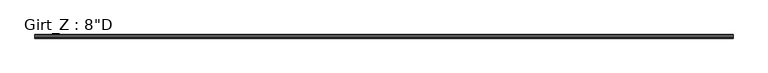
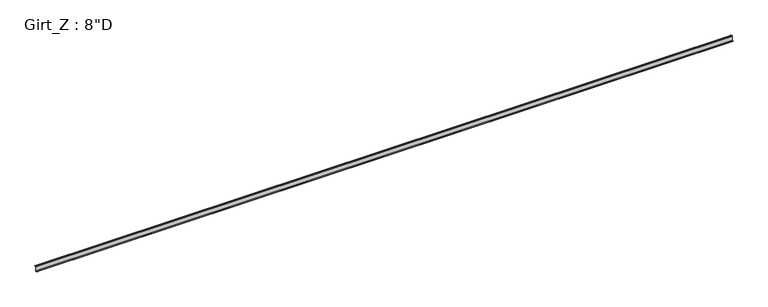
"""IFC4 building model written with IfcOpenShell, lengths in millimetres: beam geometry."""

import ifcopenshell
import ifcopenshell.guid

model = None  # the IFC model being written
_history = None  # IfcOwnerHistory: only IFC2X3 demands one
_inside = {}  # id of a spatial element -> (the spatial element, [elements in it])
_under = {}  # id of a project, library or spatial element -> (it, [spatial elements below it])
_declared = {}  # id of a project -> (the project, [libraries it declares])
_typed = {}  # id of a type object -> (the type object, [elements of that type])
_made_of = {}  # id of a material, layer set ... -> (it, [elements and type objects made of it])


def new_model(schema):
    """Start an empty IFC model of exactly this schema.

    Asked for "IFC4X3", IfcOpenShell would pick the latest addendum, in which some entities
    have other attributes; the version numbers below select the first issue.
    IFC2X3 requires an IfcOwnerHistory on every rooted entity: one is made here for all.
    """
    global model, _history
    if schema == "IFC4X3":
        model = ifcopenshell.file(schema_version=(4, 3, 0, 0))
    else:
        model = ifcopenshell.file(schema=schema)
    _inside.clear()
    _under.clear()
    _declared.clear()
    _typed.clear()
    _made_of.clear()
    _history = None
    if model.schema == "IFC2X3":
        org = make("IfcOrganization", Name="unknown")
        user = make(
            "IfcPersonAndOrganization",
            ThePerson=make("IfcPerson", FamilyName="unknown"),
            TheOrganization=org,
        )
        app = make(
            "IfcApplication",
            ApplicationDeveloper=org,
            Version="unknown",
            ApplicationFullName="unknown",
            ApplicationIdentifier="unknown",
        )
        _history = make(
            "IfcOwnerHistory",
            OwningUser=user,
            OwningApplication=app,
            ChangeAction="ADDED",
            CreationDate=0,
        )
    return model


def make(cls, **values):
    """One entity of the class cls with the attributes given. An attribute that is None is left unset."""
    return model.create_entity(
        cls, **{name: value for name, value in values.items() if value is not None}
    )


def rooted(cls, **values):
    """An entity with a GlobalId (a new one), such as an element, a storey or a relation."""
    return make(cls, GlobalId=ifcopenshell.guid.new(), OwnerHistory=_history, **values)


def si_unit(unit_type, name, prefix=None):
    """IfcSIUnit, for example si_unit("LENGTHUNIT", "METRE", prefix="MILLI")."""
    return make("IfcSIUnit", UnitType=unit_type, Prefix=prefix, Name=name)


def assignment(units):
    """IfcUnitAssignment: the units of a project."""
    return None if units is None else make("IfcUnitAssignment", Units=units)


def point(xyz):
    """IfcCartesianPoint."""
    return None if xyz is None else make("IfcCartesianPoint", Coordinates=xyz)


def direction(xyz):
    """IfcDirection."""
    return None if xyz is None else make("IfcDirection", DirectionRatios=xyz)


def frame(location, z_axis=None, x_axis=None):
    """IfcAxis2Placement3D, a coordinate frame: its origin and axes. An axis left out is left unset."""
    return make(
        "IfcAxis2Placement3D",
        Location=point(location),
        Axis=direction(z_axis),
        RefDirection=direction(x_axis),
    )


def frame_2d(location, x_axis=None):
    """IfcAxis2Placement2D, a coordinate frame in the plane: its origin and x axis."""
    return make(
        "IfcAxis2Placement2D", Location=point(location), RefDirection=direction(x_axis)
    )


def origin():
    """The frame at (0, 0, 0) with its axes left unset."""
    return frame((0.0, 0.0, 0.0))


def place(relative_to, where):
    """IfcLocalPlacement: puts the frame where relative to a parent placement (None: the world)."""
    return make(
        "IfcLocalPlacement", PlacementRelTo=relative_to, RelativePlacement=where
    )


def context(
    kind, dimensions, precision=None, world=None, true_north=None, identifier=None
):
    """IfcGeometricRepresentationContext, for example the 3D "Model" context."""
    return make(
        "IfcGeometricRepresentationContext",
        ContextIdentifier=identifier,
        ContextType=kind,
        CoordinateSpaceDimension=dimensions,
        Precision=precision,
        WorldCoordinateSystem=world,
        TrueNorth=true_north,
    )


def project(units=None, contexts=None):
    """IfcProject with its units and contexts."""
    return rooted(
        "IfcProject",
        Name="project",
        RepresentationContexts=contexts,
        UnitsInContext=assignment(units),
    )


def spatial(cls, under=None, at=None, **own):
    """A site, building, storey or space (cls), placed at a placement, below another one or the project."""
    s = rooted(cls, ObjectPlacement=at, **own)
    if under is not None:
        _under.setdefault(under.id(), (under, []))[1].append(s)
    return s


def polyline(points):
    """IfcPolyline through the points."""
    return make("IfcPolyline", Points=[point(p) for p in points])


def circle_curve(where, radius):
    """IfcCircle in the frame where."""
    return make("IfcCircle", Position=where, Radius=radius)


def trimmed(basis, trim1, trim2, sense, master):
    """IfcTrimmedCurve: the piece of a basis curve between two trims."""
    return make(
        "IfcTrimmedCurve",
        BasisCurve=basis,
        Trim1=trim1,
        Trim2=trim2,
        SenseAgreement=sense,
        MasterRepresentation=master,
    )


def segment(curve, same_sense, transition):
    """IfcCompositeCurveSegment."""
    return make(
        "IfcCompositeCurveSegment",
        Transition=transition,
        SameSense=same_sense,
        ParentCurve=curve,
    )


def composite_curve(segments, self_intersect=None):
    """IfcCompositeCurve: segments joined end to end."""
    return make("IfcCompositeCurve", Segments=segments, SelfIntersect=self_intersect)


def outline(outer, holes=None, kind="AREA"):
    """IfcArbitraryClosedProfileDef: a profile drawn as a closed curve; with holes, ...WithVoids."""
    if holes is None:
        return make("IfcArbitraryClosedProfileDef", ProfileType=kind, OuterCurve=outer)
    return make(
        "IfcArbitraryProfileDefWithVoids",
        ProfileType=kind,
        OuterCurve=outer,
        InnerCurves=holes,
    )


def extrude(swept, where, along, depth):
    """IfcExtrudedAreaSolid: the profile swept, set in the frame where, extruded along a direction by depth."""
    return make(
        "IfcExtrudedAreaSolid",
        SweptArea=swept,
        Position=where,
        ExtrudedDirection=direction(along),
        Depth=depth,
    )


def shape(context_of_items, identifier, shape_type, items):
    """IfcShapeRepresentation: the items that make up one representation, for example the "Body"."""
    return make(
        "IfcShapeRepresentation",
        ContextOfItems=context_of_items,
        RepresentationIdentifier=identifier,
        RepresentationType=shape_type,
        Items=items,
    )


def source(mapping_origin, context_of_items, identifier, shape_type, items):
    """IfcRepresentationMap: a shape defined once, which mapped items show again and again."""
    return make(
        "IfcRepresentationMap",
        MappingOrigin=mapping_origin,
        MappedRepresentation=shape(context_of_items, identifier, shape_type, items),
    )


def transform(
    local_origin,
    x_axis=None,
    y_axis=None,
    z_axis=None,
    scale=None,
    scale2=None,
    scale3=None,
    uniform=True,
):
    """IfcCartesianTransformationOperator3D, or its non-uniform kind. x_axis, y_axis, z_axis: its Axis1, 2, 3."""
    if uniform:
        return make(
            "IfcCartesianTransformationOperator3D",
            Axis1=direction(x_axis),
            Axis2=direction(y_axis),
            LocalOrigin=point(local_origin),
            Scale=scale,
            Axis3=direction(z_axis),
        )
    return make(
        "IfcCartesianTransformationOperator3DnonUniform",
        Axis1=direction(x_axis),
        Axis2=direction(y_axis),
        LocalOrigin=point(local_origin),
        Scale=scale,
        Axis3=direction(z_axis),
        Scale2=scale2,
        Scale3=scale3,
    )


def mapped(mapping_source, mapping_target):
    """IfcMappedItem: shows the shape of a source again, moved by a transform."""
    return make(
        "IfcMappedItem", MappingSource=mapping_source, MappingTarget=mapping_target
    )


def made_of(thing, what):
    """Note that an element or type object is made of a material, layer set ...; save() writes the relation."""
    if what is not None:
        _made_of.setdefault(what.id(), (what, []))[1].append(thing)
    return thing


def element(
    cls,
    number,
    at=None,
    inside=None,
    cuts=None,
    type_object=None,
    material=None,
    context=None,
    identifier="Body",
    shape_type=None,
    held_by="IfcProductDefinitionShape",
    body=None,
    shapes=None,
    **own,
):
    """One element of the class cls, such as IfcWall. Its Tag is "e" and its number.

    at: its placement. inside: the storey or other place that contains it. cuts: it is an
    opening in that element (IfcRelVoidsElement). A single representation is given by context,
    identifier, shape_type and body (its items); several are given by shapes. held_by: the class
    of the entity that holds the representations. save() writes the other relations.
    """
    e = rooted(cls, Tag="e%d" % number, ObjectPlacement=at, **own)
    if body is not None:
        shapes = [shape(context, identifier, shape_type, body)]
    if shapes is not None:
        e.Representation = make(held_by, Representations=shapes)
    if inside is not None:
        _inside.setdefault(inside.id(), (inside, []))[1].append(e)
    if cuts is not None:
        rooted(
            "IfcRelVoidsElement", RelatingBuildingElement=cuts, RelatedOpeningElement=e
        )
    if type_object is not None:
        _typed.setdefault(type_object.id(), (type_object, []))[1].append(e)
    return made_of(e, material)


def aggregate(whole, parts):
    """IfcRelAggregates: a whole, such as a stair, and the parts it consists of."""
    return rooted("IfcRelAggregates", RelatingObject=whole, RelatedObjects=parts)


def save(model, path):
    """Write the relations noted so far, then the file.

    IfcRelAggregates (storeys below a building ...), IfcRelContainedInSpatialStructure (elements
    in a storey), IfcRelDefinesByType, IfcRelAssociatesMaterial and IfcRelDeclares: one each for
    every whole, place, type object, material and project.
    """
    for whole, parts in _under.values():
        aggregate(whole, parts)
    for where, things in _inside.values():
        rooted(
            "IfcRelContainedInSpatialStructure",
            RelatedElements=things,
            RelatingStructure=where,
        )
    for kind, things in _typed.values():
        rooted("IfcRelDefinesByType", RelatedObjects=things, RelatingType=kind)
    for what, things in _made_of.values():
        rooted("IfcRelAssociatesMaterial", RelatedObjects=things, RelatingMaterial=what)
    for by, libraries in _declared.values():
        rooted("IfcRelDeclares", RelatingContext=by, RelatedDefinitions=libraries)
    model.write(path)


def beam_fce96416(model_context):
    return source(origin(), model_context, "Body", "SweptSolid", [
        extrude(outline(composite_curve([segment(polyline([(63.5, 101.6), (75.745104, 87.0068534), (73.6169367, 85.221109), (62.204539, 98.821875), (3.3005807, 98.821875)]), True, "CONTINUOUS"), segment(trimmed(circle_curve(frame_2d((3.3741066, 96.8381931)), 1.9850441), [point((3.3005807, 98.821875))], [point((1.3890625, 96.8381931))], True, "CARTESIAN"), True, "CONTINUOUS"), segment(polyline([(1.3890625, 96.8381931), (1.3890625, -96.8375)]), True, "CONTINUOUS"), segment(trimmed(circle_curve(frame_2d((-3.3734375, -96.8375)), 4.7625), [point((1.3890625, -96.8375))], [point((-3.3734375, -101.6))], False, "CARTESIAN"), True, "CONTINUOUS"), segment(polyline([(-3.3734375, -101.6), (-63.5, -101.6), (-75.745104, -87.0068534), (-73.6169367, -85.221109), (-62.204539, -98.821875), (-3.2694106, -98.821875)]), True, "CONTINUOUS"), segment(trimmed(circle_curve(frame_2d((-3.3748024, -96.8389339)), 1.9857399), [point((-3.2694106, -98.821875))], [point((-1.3890625, -96.8389339))], True, "CARTESIAN"), True, "CONTINUOUS"), segment(polyline([(-1.3890625, -96.8389339), (-1.3890625, 96.8375)]), True, "CONTINUOUS"), segment(trimmed(circle_curve(frame_2d((3.3734375, 96.8375)), 4.7625), [point((-1.3890625, 96.8375))], [point((3.3734375, 101.6))], False, "CARTESIAN"), True, "CONTINUOUS"), segment(polyline([(3.3734375, 101.6), (63.5, 101.6)]), True, "CONTINUOUS")], self_intersect=False)), frame((-14711.2384766, 0.0, 0.0), z_axis=(1.0, 0.0, 0.0), x_axis=(0.0, 1.0, 0.0)), (0.0, 0.0, 1.0), 29454.2269531),
    ])


if __name__ == "__main__":
    model = new_model("IFC4")
    model_context = context("Model", 3, world=origin())
    ifc_project = project(units=[si_unit("LENGTHUNIT", "METRE", prefix="MILLI")], contexts=[model_context])
    site = spatial("IfcSite", under=ifc_project)
    building = spatial("IfcBuilding", under=site)
    placement = place(None, origin())
    beam_shape = beam_fce96416(model_context)
    element("IfcBeam", 1, ObjectType="Girt_Z : 8\"D", at=placement, inside=building, context=model_context, shape_type="MappedRepresentation", body=[
        mapped(beam_shape, transform((0.0, 0.0, 0.0), x_axis=(1.0, 0.0, 0.0), y_axis=(0.0, 1.0, 0.0), z_axis=(0.0, 0.0, 1.0))),
    ])
    save(model, "model.ifc")

# Revit data of these elements
# Type "Girt_Z : 8\"D"
#   Web_Thickness = 0' - 0 7/64"
#   Length [instance default] = 10' - 0"
#   Leg_1 = 0' - 2 1/2"
#   Height = 0' - 8"
#   Structural Material [instance default] = none
